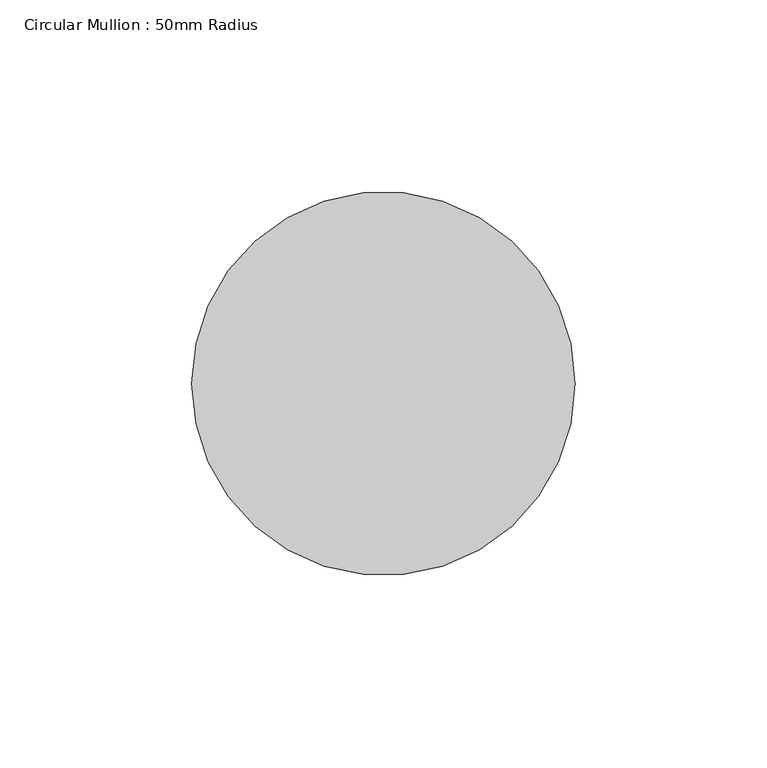
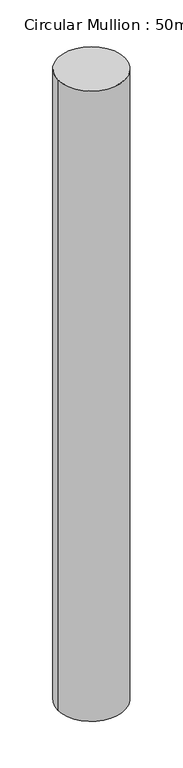
"""IFC4 building model written with IfcOpenShell, lengths in millimetres: member geometry, Circular Mullion : 50mm Radius."""

from ifc_helpers import new_model, si_unit, point, frame, origin, origin_2d, place, context, project, spatial, circle_curve, trimmed, segment, composite_curve, outline, extrude, source, transform, mapped, element, save


def circular_mullion_50mm_radius_bfad9fe6(model_context):
    return source(origin(), model_context, "Body", "SweptSolid", [
        extrude(outline(composite_curve([segment(trimmed(circle_curve(origin_2d(), 50.0), [point((50.0, 0.0))], [point((-50.0, 0.0))], False, "CARTESIAN"), True, "CONTINUOUS"), segment(trimmed(circle_curve(origin_2d(), 50.0), [point((-50.0, 0.0))], [point((50.0, 0.0))], False, "CARTESIAN"), True, "CONTINUOUS")], self_intersect=False)), frame((0.0, 0.0, -996.6802808), z_axis=(0.0, 0.0, 1.0), x_axis=(1.0, 0.0, 0.0)), (0.0, 0.0, 1.0), 996.6802808),
    ])


if __name__ == "__main__":
    model = new_model("IFC4")
    model_context = context("Model", 3, world=origin())
    ifc_project = project(units=[si_unit("LENGTHUNIT", "METRE", prefix="MILLI")], contexts=[model_context])
    site = spatial("IfcSite", under=ifc_project)
    building = spatial("IfcBuilding", under=site)
    placement = place(None, origin())
    circular_mullion_50mm_radius_shape = circular_mullion_50mm_radius_bfad9fe6(model_context)
    element("IfcMember", 1, ObjectType="Circular Mullion : 50mm Radius", at=placement, inside=building, context=model_context, shape_type="MappedRepresentation", body=[
        mapped(circular_mullion_50mm_radius_shape, transform((0.0, 0.0, 0.0), x_axis=(1.0, 0.0, 0.0), y_axis=(0.0, 1.0, 0.0), z_axis=(0.0, 0.0, 1.0))),
    ])
    save(model, "model.ifc")

# Revit data of these elements
# Type "Circular Mullion : 50mm Radius"
#   built-in parameter 1007350 = 0.164042 (stored number, unit not read)
# Element 1 (IfcMember, "Circular Mullion : 50mm Radius")
#   Materials on its faces: "Aluminium"
# Materials
#   "Aluminium": class "Metal", colour RGB 247 247 247, transparency 0, Description = "Aluminium 6061", Cost = 0
